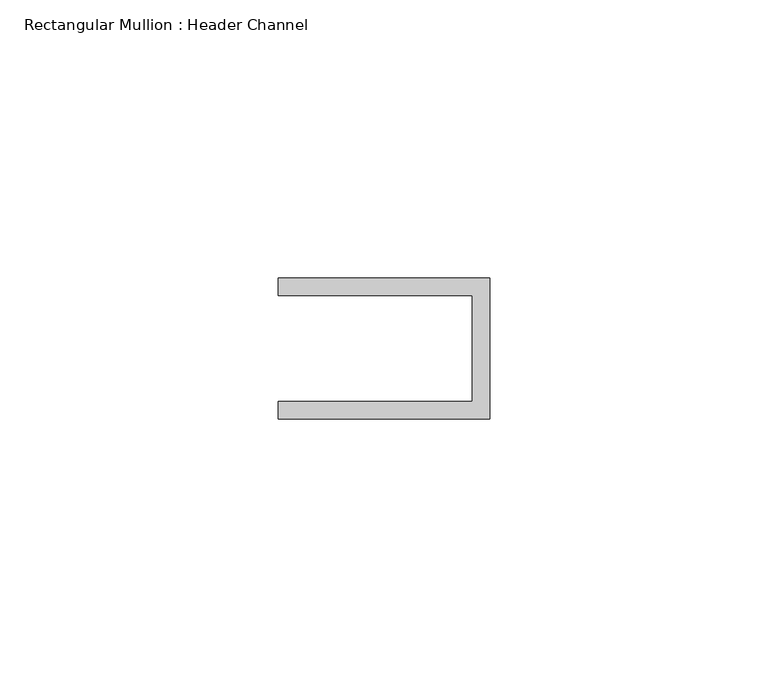
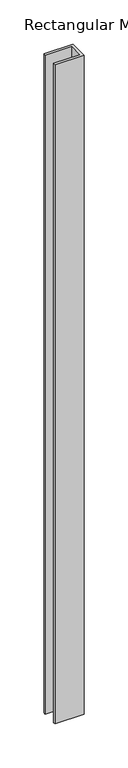
"""IFC4 building model written with IfcOpenShell, lengths in millimetres: member geometry, Rectangular Mullion : Header Channel."""

import ifcopenshell
import ifcopenshell.guid

model = None  # the IFC model being written
_history = None  # IfcOwnerHistory: only IFC2X3 demands one
_inside = {}  # id of a spatial element -> (the spatial element, [elements in it])
_under = {}  # id of a project, library or spatial element -> (it, [spatial elements below it])
_declared = {}  # id of a project -> (the project, [libraries it declares])
_typed = {}  # id of a type object -> (the type object, [elements of that type])
_made_of = {}  # id of a material, layer set ... -> (it, [elements and type objects made of it])


def new_model(schema):
    """Start an empty IFC model of exactly this schema.

    Asked for "IFC4X3", IfcOpenShell would pick the latest addendum, in which some entities
    have other attributes; the version numbers below select the first issue.
    IFC2X3 requires an IfcOwnerHistory on every rooted entity: one is made here for all.
    """
    global model, _history
    if schema == "IFC4X3":
        model = ifcopenshell.file(schema_version=(4, 3, 0, 0))
    else:
        model = ifcopenshell.file(schema=schema)
    _inside.clear()
    _under.clear()
    _declared.clear()
    _typed.clear()
    _made_of.clear()
    _history = None
    if model.schema == "IFC2X3":
        org = make("IfcOrganization", Name="unknown")
        user = make(
            "IfcPersonAndOrganization",
            ThePerson=make("IfcPerson", FamilyName="unknown"),
            TheOrganization=org,
        )
        app = make(
            "IfcApplication",
            ApplicationDeveloper=org,
            Version="unknown",
            ApplicationFullName="unknown",
            ApplicationIdentifier="unknown",
        )
        _history = make(
            "IfcOwnerHistory",
            OwningUser=user,
            OwningApplication=app,
            ChangeAction="ADDED",
            CreationDate=0,
        )
    return model


def make(cls, **values):
    """One entity of the class cls with the attributes given. An attribute that is None is left unset."""
    return model.create_entity(
        cls, **{name: value for name, value in values.items() if value is not None}
    )


def rooted(cls, **values):
    """An entity with a GlobalId (a new one), such as an element, a storey or a relation."""
    return make(cls, GlobalId=ifcopenshell.guid.new(), OwnerHistory=_history, **values)


def si_unit(unit_type, name, prefix=None):
    """IfcSIUnit, for example si_unit("LENGTHUNIT", "METRE", prefix="MILLI")."""
    return make("IfcSIUnit", UnitType=unit_type, Prefix=prefix, Name=name)


def assignment(units):
    """IfcUnitAssignment: the units of a project."""
    return None if units is None else make("IfcUnitAssignment", Units=units)


def point(xyz):
    """IfcCartesianPoint."""
    return None if xyz is None else make("IfcCartesianPoint", Coordinates=xyz)


def direction(xyz):
    """IfcDirection."""
    return None if xyz is None else make("IfcDirection", DirectionRatios=xyz)


def frame(location, z_axis=None, x_axis=None):
    """IfcAxis2Placement3D, a coordinate frame: its origin and axes. An axis left out is left unset."""
    return make(
        "IfcAxis2Placement3D",
        Location=point(location),
        Axis=direction(z_axis),
        RefDirection=direction(x_axis),
    )


def origin():
    """The frame at (0, 0, 0) with its axes left unset."""
    return frame((0.0, 0.0, 0.0))


def place(relative_to, where):
    """IfcLocalPlacement: puts the frame where relative to a parent placement (None: the world)."""
    return make(
        "IfcLocalPlacement", PlacementRelTo=relative_to, RelativePlacement=where
    )


def context(
    kind, dimensions, precision=None, world=None, true_north=None, identifier=None
):
    """IfcGeometricRepresentationContext, for example the 3D "Model" context."""
    return make(
        "IfcGeometricRepresentationContext",
        ContextIdentifier=identifier,
        ContextType=kind,
        CoordinateSpaceDimension=dimensions,
        Precision=precision,
        WorldCoordinateSystem=world,
        TrueNorth=true_north,
    )


def project(units=None, contexts=None):
    """IfcProject with its units and contexts."""
    return rooted(
        "IfcProject",
        Name="project",
        RepresentationContexts=contexts,
        UnitsInContext=assignment(units),
    )


def spatial(cls, under=None, at=None, **own):
    """A site, building, storey or space (cls), placed at a placement, below another one or the project."""
    s = rooted(cls, ObjectPlacement=at, **own)
    if under is not None:
        _under.setdefault(under.id(), (under, []))[1].append(s)
    return s


def polyline(points):
    """IfcPolyline through the points."""
    return make("IfcPolyline", Points=[point(p) for p in points])


def outline(outer, holes=None, kind="AREA"):
    """IfcArbitraryClosedProfileDef: a profile drawn as a closed curve; with holes, ...WithVoids."""
    if holes is None:
        return make("IfcArbitraryClosedProfileDef", ProfileType=kind, OuterCurve=outer)
    return make(
        "IfcArbitraryProfileDefWithVoids",
        ProfileType=kind,
        OuterCurve=outer,
        InnerCurves=holes,
    )


def extrude(swept, where, along, depth):
    """IfcExtrudedAreaSolid: the profile swept, set in the frame where, extruded along a direction by depth."""
    return make(
        "IfcExtrudedAreaSolid",
        SweptArea=swept,
        Position=where,
        ExtrudedDirection=direction(along),
        Depth=depth,
    )


def shape(context_of_items, identifier, shape_type, items):
    """IfcShapeRepresentation: the items that make up one representation, for example the "Body"."""
    return make(
        "IfcShapeRepresentation",
        ContextOfItems=context_of_items,
        RepresentationIdentifier=identifier,
        RepresentationType=shape_type,
        Items=items,
    )


def source(mapping_origin, context_of_items, identifier, shape_type, items):
    """IfcRepresentationMap: a shape defined once, which mapped items show again and again."""
    return make(
        "IfcRepresentationMap",
        MappingOrigin=mapping_origin,
        MappedRepresentation=shape(context_of_items, identifier, shape_type, items),
    )


def transform(
    local_origin,
    x_axis=None,
    y_axis=None,
    z_axis=None,
    scale=None,
    scale2=None,
    scale3=None,
    uniform=True,
):
    """IfcCartesianTransformationOperator3D, or its non-uniform kind. x_axis, y_axis, z_axis: its Axis1, 2, 3."""
    if uniform:
        return make(
            "IfcCartesianTransformationOperator3D",
            Axis1=direction(x_axis),
            Axis2=direction(y_axis),
            LocalOrigin=point(local_origin),
            Scale=scale,
            Axis3=direction(z_axis),
        )
    return make(
        "IfcCartesianTransformationOperator3DnonUniform",
        Axis1=direction(x_axis),
        Axis2=direction(y_axis),
        LocalOrigin=point(local_origin),
        Scale=scale,
        Axis3=direction(z_axis),
        Scale2=scale2,
        Scale3=scale3,
    )


def mapped(mapping_source, mapping_target):
    """IfcMappedItem: shows the shape of a source again, moved by a transform."""
    return make(
        "IfcMappedItem", MappingSource=mapping_source, MappingTarget=mapping_target
    )


def made_of(thing, what):
    """Note that an element or type object is made of a material, layer set ...; save() writes the relation."""
    if what is not None:
        _made_of.setdefault(what.id(), (what, []))[1].append(thing)
    return thing


def element(
    cls,
    number,
    at=None,
    inside=None,
    cuts=None,
    type_object=None,
    material=None,
    context=None,
    identifier="Body",
    shape_type=None,
    held_by="IfcProductDefinitionShape",
    body=None,
    shapes=None,
    **own,
):
    """One element of the class cls, such as IfcWall. Its Tag is "e" and its number.

    at: its placement. inside: the storey or other place that contains it. cuts: it is an
    opening in that element (IfcRelVoidsElement). A single representation is given by context,
    identifier, shape_type and body (its items); several are given by shapes. held_by: the class
    of the entity that holds the representations. save() writes the other relations.
    """
    e = rooted(cls, Tag="e%d" % number, ObjectPlacement=at, **own)
    if body is not None:
        shapes = [shape(context, identifier, shape_type, body)]
    if shapes is not None:
        e.Representation = make(held_by, Representations=shapes)
    if inside is not None:
        _inside.setdefault(inside.id(), (inside, []))[1].append(e)
    if cuts is not None:
        rooted(
            "IfcRelVoidsElement", RelatingBuildingElement=cuts, RelatedOpeningElement=e
        )
    if type_object is not None:
        _typed.setdefault(type_object.id(), (type_object, []))[1].append(e)
    return made_of(e, material)


def aggregate(whole, parts):
    """IfcRelAggregates: a whole, such as a stair, and the parts it consists of."""
    return rooted("IfcRelAggregates", RelatingObject=whole, RelatedObjects=parts)


def save(model, path):
    """Write the relations noted so far, then the file.

    IfcRelAggregates (storeys below a building ...), IfcRelContainedInSpatialStructure (elements
    in a storey), IfcRelDefinesByType, IfcRelAssociatesMaterial and IfcRelDeclares: one each for
    every whole, place, type object, material and project.
    """
    for whole, parts in _under.values():
        aggregate(whole, parts)
    for where, things in _inside.values():
        rooted(
            "IfcRelContainedInSpatialStructure",
            RelatedElements=things,
            RelatingStructure=where,
        )
    for kind, things in _typed.values():
        rooted("IfcRelDefinesByType", RelatedObjects=things, RelatingType=kind)
    for what, things in _made_of.values():
        rooted("IfcRelAssociatesMaterial", RelatedObjects=things, RelatingMaterial=what)
    for by, libraries in _declared.values():
        rooted("IfcRelDeclares", RelatingContext=by, RelatedDefinitions=libraries)
    model.write(path)


def rectangular_mullion_header_channel_e41eb503(model_context):
    return source(origin(), model_context, "Body", "SweptSolid", [
        extrude(outline(polyline([(0.0, 12.7), (0.0, -12.7), (-38.1, -12.7), (-38.1, -9.525), (-3.175, -9.525), (-3.175, 9.525), (-38.1, 9.525), (-38.1, 12.7), (0.0, 12.7)])), frame((0.0, 0.0, -914.4), z_axis=(0.0, 0.0, 1.0), x_axis=(1.0, 0.0, 0.0)), (0.0, 0.0, 1.0), 914.4),
    ])


if __name__ == "__main__":
    model = new_model("IFC4")
    model_context = context("Model", 3, world=origin())
    ifc_project = project(units=[si_unit("LENGTHUNIT", "METRE", prefix="MILLI")], contexts=[model_context])
    site = spatial("IfcSite", under=ifc_project)
    building = spatial("IfcBuilding", under=site)
    placement = place(None, origin())
    rectangular_mullion_header_channel_shape = rectangular_mullion_header_channel_e41eb503(model_context)
    element("IfcMember", 1, ObjectType="Rectangular Mullion : Header Channel", at=placement, inside=building, context=model_context, shape_type="MappedRepresentation", body=[
        mapped(rectangular_mullion_header_channel_shape, transform((0.0, 0.0, 0.0), x_axis=(1.0, 0.0, 0.0), y_axis=(0.0, 1.0, 0.0), z_axis=(0.0, 0.0, 1.0))),
    ])
    save(model, "model.ifc")

# Revit data of these elements
# Type "Rectangular Mullion : Header Channel"
#   built-in parameter 1007322 = 0.0833333 (stored number, unit not read)
#   built-in parameter 1007321 = -0.03125 (stored number, unit not read)
#   built-in parameter 1007320 = 0.0416667 (stored number, unit not read)
# Element 1 (IfcMember, "Rectangular Mullion : Header Channel")
#   Materials on its faces: "ALUM"
# Materials
#   "ALUM": class "Generic", colour RGB 157 157 157, transparency 0, Cost = 0
